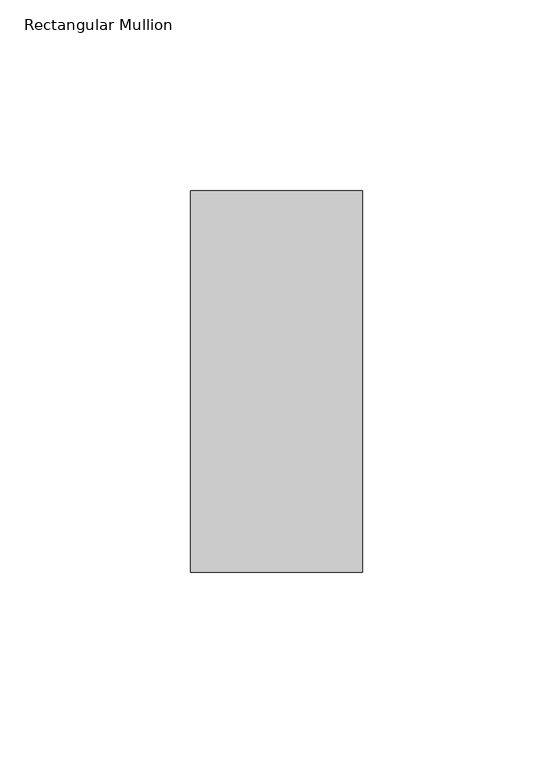
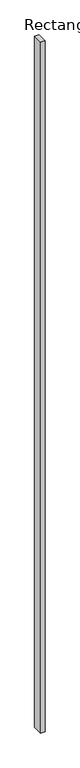
"""IFC4 building model written with IfcOpenShell, lengths in millimetres: member geometry, Rectangular Mullion : 알루미늄_Rectangular Cap_100 x 45."""

import ifcopenshell
import ifcopenshell.guid

model = None  # the IFC model being written
_history = None  # IfcOwnerHistory: only IFC2X3 demands one
_inside = {}  # id of a spatial element -> (the spatial element, [elements in it])
_under = {}  # id of a project, library or spatial element -> (it, [spatial elements below it])
_declared = {}  # id of a project -> (the project, [libraries it declares])
_typed = {}  # id of a type object -> (the type object, [elements of that type])
_made_of = {}  # id of a material, layer set ... -> (it, [elements and type objects made of it])


def new_model(schema):
    """Start an empty IFC model of exactly this schema.

    Asked for "IFC4X3", IfcOpenShell would pick the latest addendum, in which some entities
    have other attributes; the version numbers below select the first issue.
    IFC2X3 requires an IfcOwnerHistory on every rooted entity: one is made here for all.
    """
    global model, _history
    if schema == "IFC4X3":
        model = ifcopenshell.file(schema_version=(4, 3, 0, 0))
    else:
        model = ifcopenshell.file(schema=schema)
    _inside.clear()
    _under.clear()
    _declared.clear()
    _typed.clear()
    _made_of.clear()
    _history = None
    if model.schema == "IFC2X3":
        org = make("IfcOrganization", Name="unknown")
        user = make(
            "IfcPersonAndOrganization",
            ThePerson=make("IfcPerson", FamilyName="unknown"),
            TheOrganization=org,
        )
        app = make(
            "IfcApplication",
            ApplicationDeveloper=org,
            Version="unknown",
            ApplicationFullName="unknown",
            ApplicationIdentifier="unknown",
        )
        _history = make(
            "IfcOwnerHistory",
            OwningUser=user,
            OwningApplication=app,
            ChangeAction="ADDED",
            CreationDate=0,
        )
    return model


def make(cls, **values):
    """One entity of the class cls with the attributes given. An attribute that is None is left unset."""
    return model.create_entity(
        cls, **{name: value for name, value in values.items() if value is not None}
    )


def rooted(cls, **values):
    """An entity with a GlobalId (a new one), such as an element, a storey or a relation."""
    return make(cls, GlobalId=ifcopenshell.guid.new(), OwnerHistory=_history, **values)


def si_unit(unit_type, name, prefix=None):
    """IfcSIUnit, for example si_unit("LENGTHUNIT", "METRE", prefix="MILLI")."""
    return make("IfcSIUnit", UnitType=unit_type, Prefix=prefix, Name=name)


def assignment(units):
    """IfcUnitAssignment: the units of a project."""
    return None if units is None else make("IfcUnitAssignment", Units=units)


def point(xyz):
    """IfcCartesianPoint."""
    return None if xyz is None else make("IfcCartesianPoint", Coordinates=xyz)


def direction(xyz):
    """IfcDirection."""
    return None if xyz is None else make("IfcDirection", DirectionRatios=xyz)


def frame(location, z_axis=None, x_axis=None):
    """IfcAxis2Placement3D, a coordinate frame: its origin and axes. An axis left out is left unset."""
    return make(
        "IfcAxis2Placement3D",
        Location=point(location),
        Axis=direction(z_axis),
        RefDirection=direction(x_axis),
    )


def origin():
    """The frame at (0, 0, 0) with its axes left unset."""
    return frame((0.0, 0.0, 0.0))


def place(relative_to, where):
    """IfcLocalPlacement: puts the frame where relative to a parent placement (None: the world)."""
    return make(
        "IfcLocalPlacement", PlacementRelTo=relative_to, RelativePlacement=where
    )


def context(
    kind, dimensions, precision=None, world=None, true_north=None, identifier=None
):
    """IfcGeometricRepresentationContext, for example the 3D "Model" context."""
    return make(
        "IfcGeometricRepresentationContext",
        ContextIdentifier=identifier,
        ContextType=kind,
        CoordinateSpaceDimension=dimensions,
        Precision=precision,
        WorldCoordinateSystem=world,
        TrueNorth=true_north,
    )


def project(units=None, contexts=None):
    """IfcProject with its units and contexts."""
    return rooted(
        "IfcProject",
        Name="project",
        RepresentationContexts=contexts,
        UnitsInContext=assignment(units),
    )


def spatial(cls, under=None, at=None, **own):
    """A site, building, storey or space (cls), placed at a placement, below another one or the project."""
    s = rooted(cls, ObjectPlacement=at, **own)
    if under is not None:
        _under.setdefault(under.id(), (under, []))[1].append(s)
    return s


def polyline(points):
    """IfcPolyline through the points."""
    return make("IfcPolyline", Points=[point(p) for p in points])


def outline(outer, holes=None, kind="AREA"):
    """IfcArbitraryClosedProfileDef: a profile drawn as a closed curve; with holes, ...WithVoids."""
    if holes is None:
        return make("IfcArbitraryClosedProfileDef", ProfileType=kind, OuterCurve=outer)
    return make(
        "IfcArbitraryProfileDefWithVoids",
        ProfileType=kind,
        OuterCurve=outer,
        InnerCurves=holes,
    )


def extrude(swept, where, along, depth):
    """IfcExtrudedAreaSolid: the profile swept, set in the frame where, extruded along a direction by depth."""
    return make(
        "IfcExtrudedAreaSolid",
        SweptArea=swept,
        Position=where,
        ExtrudedDirection=direction(along),
        Depth=depth,
    )


def shape(context_of_items, identifier, shape_type, items):
    """IfcShapeRepresentation: the items that make up one representation, for example the "Body"."""
    return make(
        "IfcShapeRepresentation",
        ContextOfItems=context_of_items,
        RepresentationIdentifier=identifier,
        RepresentationType=shape_type,
        Items=items,
    )


def source(mapping_origin, context_of_items, identifier, shape_type, items):
    """IfcRepresentationMap: a shape defined once, which mapped items show again and again."""
    return make(
        "IfcRepresentationMap",
        MappingOrigin=mapping_origin,
        MappedRepresentation=shape(context_of_items, identifier, shape_type, items),
    )


def transform(
    local_origin,
    x_axis=None,
    y_axis=None,
    z_axis=None,
    scale=None,
    scale2=None,
    scale3=None,
    uniform=True,
):
    """IfcCartesianTransformationOperator3D, or its non-uniform kind. x_axis, y_axis, z_axis: its Axis1, 2, 3."""
    if uniform:
        return make(
            "IfcCartesianTransformationOperator3D",
            Axis1=direction(x_axis),
            Axis2=direction(y_axis),
            LocalOrigin=point(local_origin),
            Scale=scale,
            Axis3=direction(z_axis),
        )
    return make(
        "IfcCartesianTransformationOperator3DnonUniform",
        Axis1=direction(x_axis),
        Axis2=direction(y_axis),
        LocalOrigin=point(local_origin),
        Scale=scale,
        Axis3=direction(z_axis),
        Scale2=scale2,
        Scale3=scale3,
    )


def mapped(mapping_source, mapping_target):
    """IfcMappedItem: shows the shape of a source again, moved by a transform."""
    return make(
        "IfcMappedItem", MappingSource=mapping_source, MappingTarget=mapping_target
    )


def made_of(thing, what):
    """Note that an element or type object is made of a material, layer set ...; save() writes the relation."""
    if what is not None:
        _made_of.setdefault(what.id(), (what, []))[1].append(thing)
    return thing


def element(
    cls,
    number,
    at=None,
    inside=None,
    cuts=None,
    type_object=None,
    material=None,
    context=None,
    identifier="Body",
    shape_type=None,
    held_by="IfcProductDefinitionShape",
    body=None,
    shapes=None,
    **own,
):
    """One element of the class cls, such as IfcWall. Its Tag is "e" and its number.

    at: its placement. inside: the storey or other place that contains it. cuts: it is an
    opening in that element (IfcRelVoidsElement). A single representation is given by context,
    identifier, shape_type and body (its items); several are given by shapes. held_by: the class
    of the entity that holds the representations. save() writes the other relations.
    """
    e = rooted(cls, Tag="e%d" % number, ObjectPlacement=at, **own)
    if body is not None:
        shapes = [shape(context, identifier, shape_type, body)]
    if shapes is not None:
        e.Representation = make(held_by, Representations=shapes)
    if inside is not None:
        _inside.setdefault(inside.id(), (inside, []))[1].append(e)
    if cuts is not None:
        rooted(
            "IfcRelVoidsElement", RelatingBuildingElement=cuts, RelatedOpeningElement=e
        )
    if type_object is not None:
        _typed.setdefault(type_object.id(), (type_object, []))[1].append(e)
    return made_of(e, material)


def aggregate(whole, parts):
    """IfcRelAggregates: a whole, such as a stair, and the parts it consists of."""
    return rooted("IfcRelAggregates", RelatingObject=whole, RelatedObjects=parts)


def save(model, path):
    """Write the relations noted so far, then the file.

    IfcRelAggregates (storeys below a building ...), IfcRelContainedInSpatialStructure (elements
    in a storey), IfcRelDefinesByType, IfcRelAssociatesMaterial and IfcRelDeclares: one each for
    every whole, place, type object, material and project.
    """
    for whole, parts in _under.values():
        aggregate(whole, parts)
    for where, things in _inside.values():
        rooted(
            "IfcRelContainedInSpatialStructure",
            RelatedElements=things,
            RelatingStructure=where,
        )
    for kind, things in _typed.values():
        rooted("IfcRelDefinesByType", RelatedObjects=things, RelatingType=kind)
    for what, things in _made_of.values():
        rooted("IfcRelAssociatesMaterial", RelatedObjects=things, RelatingMaterial=what)
    for by, libraries in _declared.values():
        rooted("IfcRelDeclares", RelatingContext=by, RelatedDefinitions=libraries)
    model.write(path)


def rectangular_mullion_c7b7c2a1(model_context):
    return source(origin(), model_context, "Body", "SweptSolid", [
        extrude(outline(polyline([(0.0, 50.0), (0.0, -50.0), (-45.0, -50.0), (-45.0, 50.0), (0.0, 50.0)])), frame((0.0, 0.0, -7160.0000001), z_axis=(0.0, 0.0, 1.0), x_axis=(1.0, 0.0, 0.0)), (0.0, 0.0, 1.0), 7160.0000001),
    ])


if __name__ == "__main__":
    model = new_model("IFC4")
    model_context = context("Model", 3, world=origin())
    ifc_project = project(units=[si_unit("LENGTHUNIT", "METRE", prefix="MILLI")], contexts=[model_context])
    site = spatial("IfcSite", under=ifc_project)
    building = spatial("IfcBuilding", under=site)
    placement = place(None, origin())
    rectangular_mullion_shape = rectangular_mullion_c7b7c2a1(model_context)
    element("IfcMember", 1, ObjectType="Rectangular Mullion : 알루미늄_Rectangular Cap_100 x 45", at=placement, inside=building, context=model_context, shape_type="MappedRepresentation", body=[
        mapped(rectangular_mullion_shape, transform((0.0, 0.0, 0.0), x_axis=(1.0, 0.0, 0.0), y_axis=(0.0, 1.0, 0.0), z_axis=(0.0, 0.0, 1.0))),
    ])
    save(model, "model.ifc")

# Revit data of these elements
# Type "Rectangular Mullion : 알루미늄_Rectangular Cap_100 x 45"
#   built-in parameter 1007304 = 0.328084 (stored number, unit not read)
#   built-in parameter 1007301 = 0.0738189 (stored number, unit not read)
#   built-in parameter 1007300 = 0.0738189 (stored number, unit not read)
# Element 1 (IfcMember, "Rectangular Mullion : 알루미늄_Rectangular Cap_100 x 45")
#   Materials on its faces: "00_Metal_Stainless Steel"
# Materials
#   "00_Metal_Stainless Steel": class "Metal", colour RGB 148 148 148, transparency 0, Description = "Steel", Cost = 0
